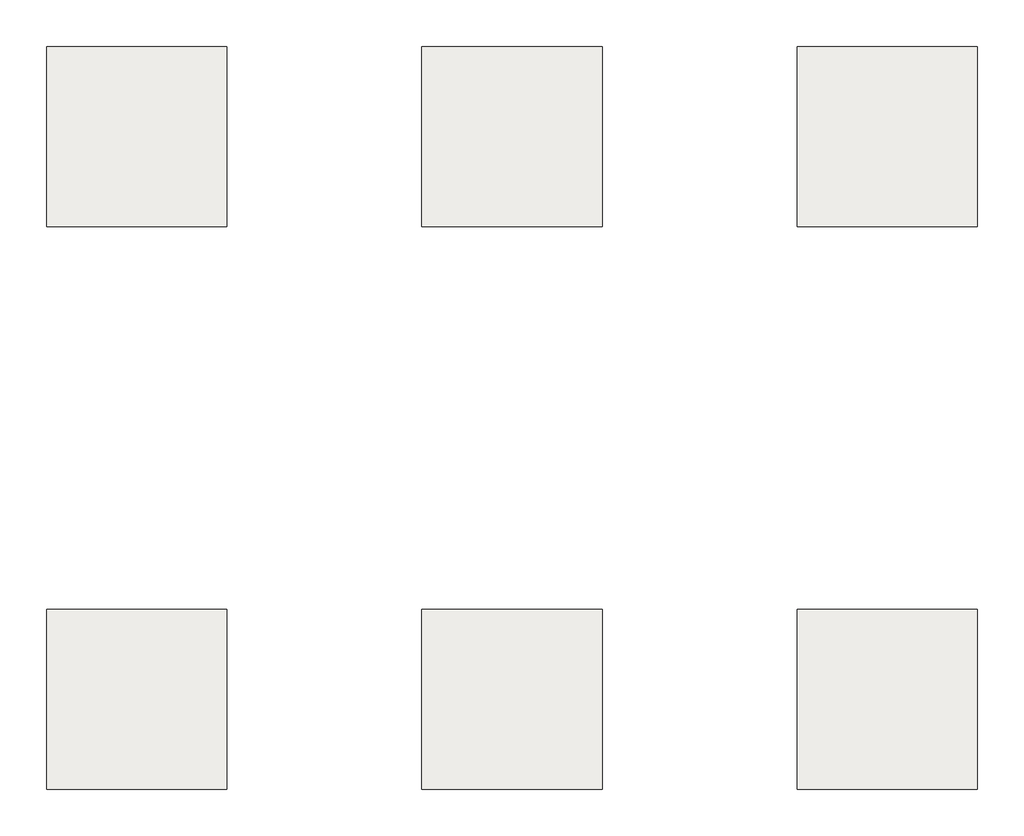
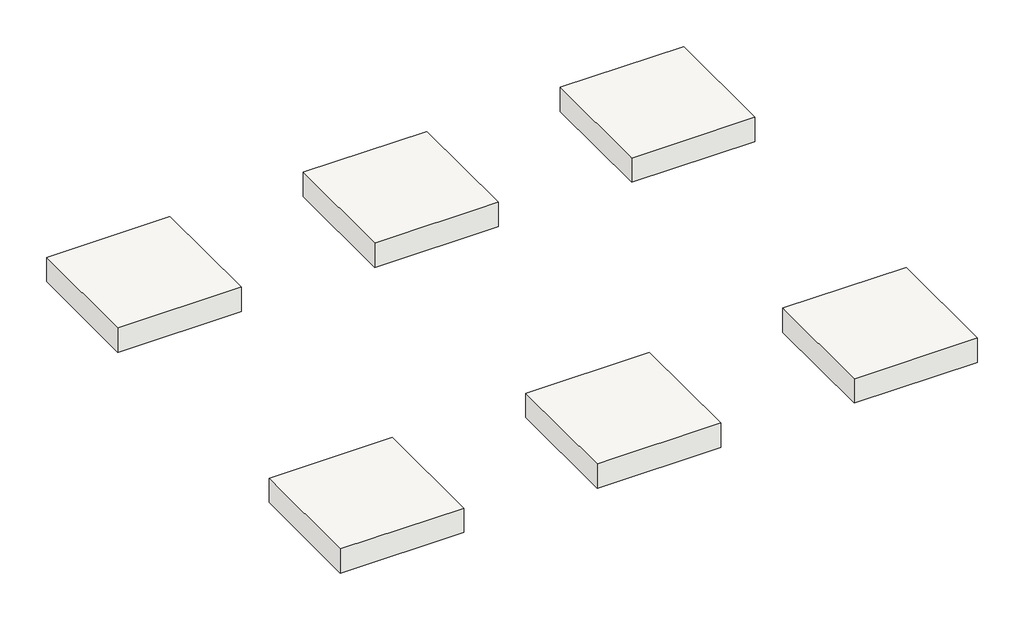
# Not in any storey: 6 slabs.
"""IFC4 building model written with IfcOpenShell, lengths in millimetres."""

import ifcopenshell
import ifcopenshell.guid

model = None  # the IFC model being written
_history = None  # IfcOwnerHistory: only IFC2X3 demands one
_inside = {}  # id of a spatial element -> (the spatial element, [elements in it])
_under = {}  # id of a project, library or spatial element -> (it, [spatial elements below it])
_declared = {}  # id of a project -> (the project, [libraries it declares])
_typed = {}  # id of a type object -> (the type object, [elements of that type])
_made_of = {}  # id of a material, layer set ... -> (it, [elements and type objects made of it])


def new_model(schema):
    """Start an empty IFC model of exactly this schema.

    Asked for "IFC4X3", IfcOpenShell would pick the latest addendum, in which some entities
    have other attributes; the version numbers below select the first issue.
    IFC2X3 requires an IfcOwnerHistory on every rooted entity: one is made here for all.
    """
    global model, _history
    if schema == "IFC4X3":
        model = ifcopenshell.file(schema_version=(4, 3, 0, 0))
    else:
        model = ifcopenshell.file(schema=schema)
    _inside.clear()
    _under.clear()
    _declared.clear()
    _typed.clear()
    _made_of.clear()
    _history = None
    if model.schema == "IFC2X3":
        org = make("IfcOrganization", Name="unknown")
        user = make(
            "IfcPersonAndOrganization",
            ThePerson=make("IfcPerson", FamilyName="unknown"),
            TheOrganization=org,
        )
        app = make(
            "IfcApplication",
            ApplicationDeveloper=org,
            Version="unknown",
            ApplicationFullName="unknown",
            ApplicationIdentifier="unknown",
        )
        _history = make(
            "IfcOwnerHistory",
            OwningUser=user,
            OwningApplication=app,
            ChangeAction="ADDED",
            CreationDate=0,
        )
    return model


def make(cls, **values):
    """One entity of the class cls with the attributes given. An attribute that is None is left unset."""
    return model.create_entity(
        cls, **{name: value for name, value in values.items() if value is not None}
    )


def rooted(cls, **values):
    """An entity with a GlobalId (a new one), such as an element, a storey or a relation."""
    return make(cls, GlobalId=ifcopenshell.guid.new(), OwnerHistory=_history, **values)


def si_unit(unit_type, name, prefix=None):
    """IfcSIUnit, for example si_unit("LENGTHUNIT", "METRE", prefix="MILLI")."""
    return make("IfcSIUnit", UnitType=unit_type, Prefix=prefix, Name=name)


def assignment(units):
    """IfcUnitAssignment: the units of a project."""
    return None if units is None else make("IfcUnitAssignment", Units=units)


def point(xyz):
    """IfcCartesianPoint."""
    return None if xyz is None else make("IfcCartesianPoint", Coordinates=xyz)


def direction(xyz):
    """IfcDirection."""
    return None if xyz is None else make("IfcDirection", DirectionRatios=xyz)


def frame(location, z_axis=None, x_axis=None):
    """IfcAxis2Placement3D, a coordinate frame: its origin and axes. An axis left out is left unset."""
    return make(
        "IfcAxis2Placement3D",
        Location=point(location),
        Axis=direction(z_axis),
        RefDirection=direction(x_axis),
    )


def origin():
    """The frame at (0, 0, 0) with its axes left unset."""
    return frame((0.0, 0.0, 0.0))


def place(relative_to, where):
    """IfcLocalPlacement: puts the frame where relative to a parent placement (None: the world)."""
    return make(
        "IfcLocalPlacement", PlacementRelTo=relative_to, RelativePlacement=where
    )


def context(
    kind, dimensions, precision=None, world=None, true_north=None, identifier=None
):
    """IfcGeometricRepresentationContext, for example the 3D "Model" context."""
    return make(
        "IfcGeometricRepresentationContext",
        ContextIdentifier=identifier,
        ContextType=kind,
        CoordinateSpaceDimension=dimensions,
        Precision=precision,
        WorldCoordinateSystem=world,
        TrueNorth=true_north,
    )


def project(units=None, contexts=None):
    """IfcProject with its units and contexts."""
    return rooted(
        "IfcProject",
        Name="project",
        RepresentationContexts=contexts,
        UnitsInContext=assignment(units),
    )


def spatial(cls, under=None, at=None, **own):
    """A site, building, storey or space (cls), placed at a placement, below another one or the project."""
    s = rooted(cls, ObjectPlacement=at, **own)
    if under is not None:
        _under.setdefault(under.id(), (under, []))[1].append(s)
    return s


def polyline(points):
    """IfcPolyline through the points."""
    return make("IfcPolyline", Points=[point(p) for p in points])


def outline(outer, holes=None, kind="AREA"):
    """IfcArbitraryClosedProfileDef: a profile drawn as a closed curve; with holes, ...WithVoids."""
    if holes is None:
        return make("IfcArbitraryClosedProfileDef", ProfileType=kind, OuterCurve=outer)
    return make(
        "IfcArbitraryProfileDefWithVoids",
        ProfileType=kind,
        OuterCurve=outer,
        InnerCurves=holes,
    )


def extrude(swept, where, along, depth):
    """IfcExtrudedAreaSolid: the profile swept, set in the frame where, extruded along a direction by depth."""
    return make(
        "IfcExtrudedAreaSolid",
        SweptArea=swept,
        Position=where,
        ExtrudedDirection=direction(along),
        Depth=depth,
    )


def shape(context_of_items, identifier, shape_type, items):
    """IfcShapeRepresentation: the items that make up one representation, for example the "Body"."""
    return make(
        "IfcShapeRepresentation",
        ContextOfItems=context_of_items,
        RepresentationIdentifier=identifier,
        RepresentationType=shape_type,
        Items=items,
    )


def made_of(thing, what):
    """Note that an element or type object is made of a material, layer set ...; save() writes the relation."""
    if what is not None:
        _made_of.setdefault(what.id(), (what, []))[1].append(thing)
    return thing


def element(
    cls,
    number,
    at=None,
    inside=None,
    cuts=None,
    type_object=None,
    material=None,
    context=None,
    identifier="Body",
    shape_type=None,
    held_by="IfcProductDefinitionShape",
    body=None,
    shapes=None,
    **own,
):
    """One element of the class cls, such as IfcWall. Its Tag is "e" and its number.

    at: its placement. inside: the storey or other place that contains it. cuts: it is an
    opening in that element (IfcRelVoidsElement). A single representation is given by context,
    identifier, shape_type and body (its items); several are given by shapes. held_by: the class
    of the entity that holds the representations. save() writes the other relations.
    """
    e = rooted(cls, Tag="e%d" % number, ObjectPlacement=at, **own)
    if body is not None:
        shapes = [shape(context, identifier, shape_type, body)]
    if shapes is not None:
        e.Representation = make(held_by, Representations=shapes)
    if inside is not None:
        _inside.setdefault(inside.id(), (inside, []))[1].append(e)
    if cuts is not None:
        rooted(
            "IfcRelVoidsElement", RelatingBuildingElement=cuts, RelatedOpeningElement=e
        )
    if type_object is not None:
        _typed.setdefault(type_object.id(), (type_object, []))[1].append(e)
    return made_of(e, material)


def aggregate(whole, parts):
    """IfcRelAggregates: a whole, such as a stair, and the parts it consists of."""
    return rooted("IfcRelAggregates", RelatingObject=whole, RelatedObjects=parts)


def save(model, path):
    """Write the relations noted so far, then the file.

    IfcRelAggregates (storeys below a building ...), IfcRelContainedInSpatialStructure (elements
    in a storey), IfcRelDefinesByType, IfcRelAssociatesMaterial and IfcRelDeclares: one each for
    every whole, place, type object, material and project.
    """
    for whole, parts in _under.values():
        aggregate(whole, parts)
    for where, things in _inside.values():
        rooted(
            "IfcRelContainedInSpatialStructure",
            RelatedElements=things,
            RelatingStructure=where,
        )
    for kind, things in _typed.values():
        rooted("IfcRelDefinesByType", RelatedObjects=things, RelatingType=kind)
    for what, things in _made_of.values():
        rooted("IfcRelAssociatesMaterial", RelatedObjects=things, RelatingMaterial=what)
    for by, libraries in _declared.values():
        rooted("IfcRelDeclares", RelatingContext=by, RelatedDefinitions=libraries)
    model.write(path)


model = new_model("IFC4")

# Units and contexts
model_context = context("Model", 3, world=origin())
ifc_project = project(units=[si_unit("LENGTHUNIT", "METRE", prefix="MILLI")], contexts=[model_context])

# Site, building
site = spatial("IfcSite", under=ifc_project)
building = spatial("IfcBuilding", under=site)

# Slabs
placement = place(None, origin())
element("IfcSlab", 1, ObjectType="FT211-Footing-Rectangular_더미삭제 : FT211_2400x2400x500", at=placement, inside=building, context=model_context, shape_type="SweptSolid", body=[
    extrude(outline(polyline([(6200.0, 14699.5208589), (6200.0, 12299.5208589), (3800.0, 12299.5208589), (3800.0, 14699.5208589), (6200.0, 14699.5208589)])), frame((0.0, 0.0, -1800.0), z_axis=(0.0, 0.0, 1.0), x_axis=(1.0, 0.0, 0.0)), (0.0, 0.0, 1.0), 500.0),
])
element("IfcSlab", 2, ObjectType="FT211-Footing-Rectangular_더미삭제 : FT211_2400x2400x500", at=placement, inside=building, context=model_context, shape_type="SweptSolid", body=[
    extrude(outline(polyline([(11200.0, 14699.5208589), (11200.0, 12299.5208589), (8800.0, 12299.5208589), (8800.0, 14699.5208589), (11200.0, 14699.5208589)])), frame((0.0, 0.0, -1800.0), z_axis=(0.0, 0.0, 1.0), x_axis=(1.0, 0.0, 0.0)), (0.0, 0.0, 1.0), 500.0),
])
element("IfcSlab", 3, ObjectType="FT211-Footing-Rectangular_더미삭제 : FT211_2400x2400x500", at=placement, inside=building, context=model_context, shape_type="SweptSolid", body=[
    extrude(outline(polyline([(11200.0, 22199.5208589), (11200.0, 19799.5208589), (8800.0, 19799.5208589), (8800.0, 22199.5208589), (11200.0, 22199.5208589)])), frame((0.0, 0.0, -1800.0), z_axis=(0.0, 0.0, 1.0), x_axis=(1.0, 0.0, 0.0)), (0.0, 0.0, 1.0), 500.0),
])
element("IfcSlab", 4, ObjectType="FT211-Footing-Rectangular_더미삭제 : FT211_2400x2400x500", at=placement, inside=building, context=model_context, shape_type="SweptSolid", body=[
    extrude(outline(polyline([(6200.0, 22199.5208589), (6200.0, 19799.5208589), (3800.0, 19799.5208589), (3800.0, 22199.5208589), (6200.0, 22199.5208589)])), frame((0.0, 0.0, -1800.0), z_axis=(0.0, 0.0, 1.0), x_axis=(1.0, 0.0, 0.0)), (0.0, 0.0, 1.0), 500.0),
])
element("IfcSlab", 5, ObjectType="FT211-Footing-Rectangular_더미삭제 : FT211_2400x2400x500", at=placement, inside=building, context=model_context, shape_type="SweptSolid", body=[
    extrude(outline(polyline([(1200.0, 22199.5208589), (1200.0, 19799.5208589), (-1200.0, 19799.5208589), (-1200.0, 22199.5208589), (1200.0, 22199.5208589)])), frame((0.0, 0.0, -1800.0), z_axis=(0.0, 0.0, 1.0), x_axis=(1.0, 0.0, 0.0)), (0.0, 0.0, 1.0), 500.0),
])
element("IfcSlab", 6, ObjectType="FT211-Footing-Rectangular_더미삭제 : FT211_2400x2400x500", at=placement, inside=building, context=model_context, shape_type="SweptSolid", body=[
    extrude(outline(polyline([(1200.0, 14699.5208589), (1200.0, 12299.5208589), (-1200.0, 12299.5208589), (-1200.0, 14699.5208589), (1200.0, 14699.5208589)])), frame((0.0, 0.0, -1800.0), z_axis=(0.0, 0.0, 1.0), x_axis=(1.0, 0.0, 0.0)), (0.0, 0.0, 1.0), 500.0),
])

save(model, "model.ifc")

# Revit data of these elements
# Project information
#   Building Name = "MAIN GATE SECURITY BUILDING"
#   Project Status = "Project Status"
#   Client Name = "현대엔지니어링"
#   Project Address = "서울시 종로구 율곡로 75(계동)"
#   Project Name = "Therma Visayas Energy Project"
#   Project Number = "-"
# Grids (mm)
#   "A": line (0, 24502.793) -> (0, 11308.625)
#   "B": line (5000, 24502.793) -> (5000, 11308.625)
#   "C": line (10000, 24502.793) -> (10000, 11308.625)
#   "1": line (-3860.098, 13499.521) -> (12441.468, 13499.521)
#   "2": line (-3860.098, 20999.521) -> (12441.468, 20999.521)
# Type "FT211-Footing-Rectangular_더미삭제 : FT211_2400x2400x500"
#   Top bar = "D25@300"
#   Description = "UG Shallow Foundation"
#   Bottom bar = "D20@300"
#   Width = 2400 mm
#   Length = 2400 mm
#   Foundation Thickness = 500 mm
#   Structural Material [instance default] = A03AC032-00007_Structural Concrete_Type1_25MPa-30Mpa
#   Assembly Code = ""
# Elements 1, 2, 3, 4, 5, 6 (IfcSlab, "FT211-Footing-Rectangular_더미삭제 : FT211_2400x2400x500")
#   Comments = ""
#   Mark = "F1"
#   F01) Building Name = "Main Gate House"
#   F11) Project Building Tag_Type-1 = "Common"
#   F12) Project Building Tag_Type-2 = "Common"
#   F13) Project Facility Code = "Facility Code"
#   F21) Structural Type = "Concrete"
#   F31) Standard Building Code = "IBC"
#   F41) Discipline = "AR"
#   F51) Plan Start Date-Engineering = "2015-01-01"
#   F52) Plan Finish Date-Engineering = "2015-12-31"
#   F53) Duration = "365"
#   F54) Actual Start Date-Engineering = "2015-01-01"
#   F55) Actual Finish Date-Engineering = "2015-12-31"
#   F61) Plan Start Date-Construction = "2016-08-19"
#   F62) Plan Finish Date-Construction = "2017-01-31"
#   F64) Actual Start Date-Construction = "2016-08-19"
#   F63) Duration = "202"
#   F65) Actual Finish Date-Construction = "2017-01-31"
#   F91) Plant Type = "CFPP"
#   F92) KKS Structures, Building = "UYF"
#   P01) Project Name = "TVEP"
#   P02) Project Configuration = "CFB Boiler x 2(Foster Wheeler) + STG x 2(Alstom, 150MW)"
#   P03) Project Abbreviation = "TVEP"
#   P04) Project Code = "BEPH1402"
#   P05) Project Stage = "In operation"
#   P06) Project Location = "Sito Looc, Barangay Bato, Toledo City in Philippines"
#   P07) Project Owner = "Therma Visayas, Inc."
#   P08) Project O.E = "Flour"
#   P09) Project Schedule = "ITB Issueing Date : 2013.07.30\r\nSite Survey : 2013.08.19-20\r\nBid Closing Date : 2013.11.29\r\nPreferred Bidder Notice 접수 : 2014.04.27\r\nTarget award date : 2014 05\r\nLOA 접수 : 2014.05.21\r\nSigning Ceremony : 2014.05.30"
#   P10) Basic Wind Speed = "55.6 m/s"
#   P11) Seismic = "NSCP 2010, Zone 4 (PGA : 0.4g)"
#   P12) Soil = "Sc"
#   P13) Soil Capacity = "100kN/m2"
#   P14) Pile Capacity = "PHC(D400) : 1200kN"
#   W00) Work Master Code = "A03AC032-00007"
#   W01) Work Master_Lv1 = "Concrete Work"
#   W02) Work Master_Lv2 = "Substructure Work"
#   W03) Work Master_Spec.1 = "Cement Type-1"
#   W04) Work Master_Spec.2 = "25MPa < F'c (Cylinder Strength) ≤ 30MPa"
#   W11) Activity ID = "C02AGB010"
#   W12) Activity Name = "Main Gate Security Building - Building Foundation"
#   W13) Plan Start Date = "2016-08-19"
#   W14) Plan Finish Date = "2016-09-22"
#   W15) Duration = "26"
#   W16) Actual Start Date = "2016-08-19"
#   W17) Actual Finish Date = "2016-09-22"
#   R02) Unit Price = 0
#   Structural Material = A03AC032-00007_Structural Concrete_Type1_25MPa-30Mpa
#   Phase Created = New Construction
#   Materials on its faces: "A03AC032-00007_Structural Concrete_Type1_25MPa-30Mpa"
# Materials
#   "A03AC032-00007_Structural Concrete_Type1_25MPa-30Mpa": class "Concrete", colour RGB 176 176 176, transparency 0, Keynote = "09910.A1", Description = "Reinf. Conc.", W00) Work Master Code = "A03AC032-00007", W01) Work Master_Lv1 = "Concrete Work", W02) Work Master_Lv2 = "Substructure Work", W03) Work Master_Spec.1 = "Structural Concrete", W04) Work Master_Spec.2 = "Cement Type-1", W05) Work Master_Spec.3 = "25MPa < F'c (Cylinder Strength) ≤ 30MPa", Cost = 0
